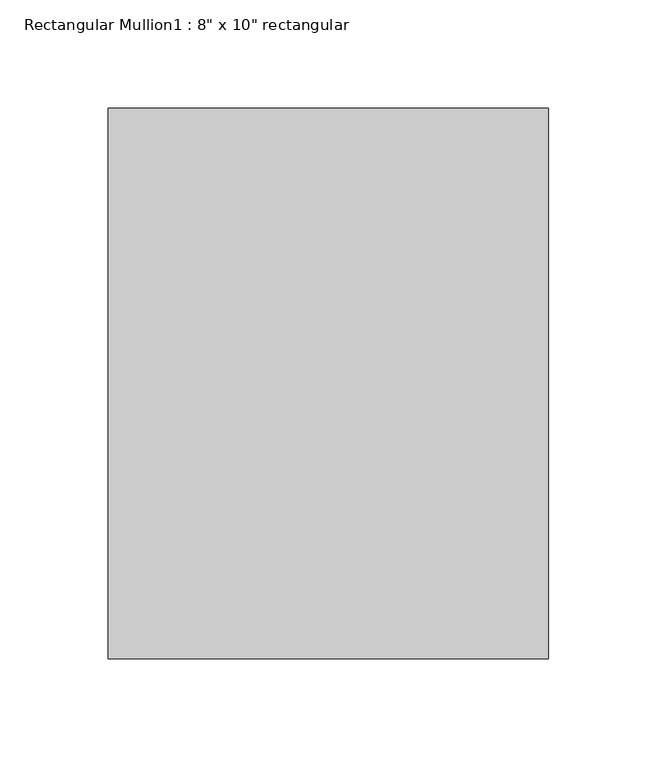
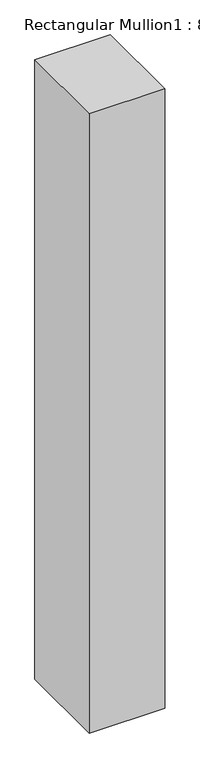
"""IFC4 building model written with IfcOpenShell, lengths in millimetres: member geometry."""

import ifcopenshell
import ifcopenshell.guid

model = None  # the IFC model being written
_history = None  # IfcOwnerHistory: only IFC2X3 demands one
_inside = {}  # id of a spatial element -> (the spatial element, [elements in it])
_under = {}  # id of a project, library or spatial element -> (it, [spatial elements below it])
_declared = {}  # id of a project -> (the project, [libraries it declares])
_typed = {}  # id of a type object -> (the type object, [elements of that type])
_made_of = {}  # id of a material, layer set ... -> (it, [elements and type objects made of it])


def new_model(schema):
    """Start an empty IFC model of exactly this schema.

    Asked for "IFC4X3", IfcOpenShell would pick the latest addendum, in which some entities
    have other attributes; the version numbers below select the first issue.
    IFC2X3 requires an IfcOwnerHistory on every rooted entity: one is made here for all.
    """
    global model, _history
    if schema == "IFC4X3":
        model = ifcopenshell.file(schema_version=(4, 3, 0, 0))
    else:
        model = ifcopenshell.file(schema=schema)
    _inside.clear()
    _under.clear()
    _declared.clear()
    _typed.clear()
    _made_of.clear()
    _history = None
    if model.schema == "IFC2X3":
        org = make("IfcOrganization", Name="unknown")
        user = make(
            "IfcPersonAndOrganization",
            ThePerson=make("IfcPerson", FamilyName="unknown"),
            TheOrganization=org,
        )
        app = make(
            "IfcApplication",
            ApplicationDeveloper=org,
            Version="unknown",
            ApplicationFullName="unknown",
            ApplicationIdentifier="unknown",
        )
        _history = make(
            "IfcOwnerHistory",
            OwningUser=user,
            OwningApplication=app,
            ChangeAction="ADDED",
            CreationDate=0,
        )
    return model


def make(cls, **values):
    """One entity of the class cls with the attributes given. An attribute that is None is left unset."""
    return model.create_entity(
        cls, **{name: value for name, value in values.items() if value is not None}
    )


def rooted(cls, **values):
    """An entity with a GlobalId (a new one), such as an element, a storey or a relation."""
    return make(cls, GlobalId=ifcopenshell.guid.new(), OwnerHistory=_history, **values)


def si_unit(unit_type, name, prefix=None):
    """IfcSIUnit, for example si_unit("LENGTHUNIT", "METRE", prefix="MILLI")."""
    return make("IfcSIUnit", UnitType=unit_type, Prefix=prefix, Name=name)


def assignment(units):
    """IfcUnitAssignment: the units of a project."""
    return None if units is None else make("IfcUnitAssignment", Units=units)


def point(xyz):
    """IfcCartesianPoint."""
    return None if xyz is None else make("IfcCartesianPoint", Coordinates=xyz)


def direction(xyz):
    """IfcDirection."""
    return None if xyz is None else make("IfcDirection", DirectionRatios=xyz)


def frame(location, z_axis=None, x_axis=None):
    """IfcAxis2Placement3D, a coordinate frame: its origin and axes. An axis left out is left unset."""
    return make(
        "IfcAxis2Placement3D",
        Location=point(location),
        Axis=direction(z_axis),
        RefDirection=direction(x_axis),
    )


def origin():
    """The frame at (0, 0, 0) with its axes left unset."""
    return frame((0.0, 0.0, 0.0))


def place(relative_to, where):
    """IfcLocalPlacement: puts the frame where relative to a parent placement (None: the world)."""
    return make(
        "IfcLocalPlacement", PlacementRelTo=relative_to, RelativePlacement=where
    )


def context(
    kind, dimensions, precision=None, world=None, true_north=None, identifier=None
):
    """IfcGeometricRepresentationContext, for example the 3D "Model" context."""
    return make(
        "IfcGeometricRepresentationContext",
        ContextIdentifier=identifier,
        ContextType=kind,
        CoordinateSpaceDimension=dimensions,
        Precision=precision,
        WorldCoordinateSystem=world,
        TrueNorth=true_north,
    )


def project(units=None, contexts=None):
    """IfcProject with its units and contexts."""
    return rooted(
        "IfcProject",
        Name="project",
        RepresentationContexts=contexts,
        UnitsInContext=assignment(units),
    )


def spatial(cls, under=None, at=None, **own):
    """A site, building, storey or space (cls), placed at a placement, below another one or the project."""
    s = rooted(cls, ObjectPlacement=at, **own)
    if under is not None:
        _under.setdefault(under.id(), (under, []))[1].append(s)
    return s


def polyline(points):
    """IfcPolyline through the points."""
    return make("IfcPolyline", Points=[point(p) for p in points])


def outline(outer, holes=None, kind="AREA"):
    """IfcArbitraryClosedProfileDef: a profile drawn as a closed curve; with holes, ...WithVoids."""
    if holes is None:
        return make("IfcArbitraryClosedProfileDef", ProfileType=kind, OuterCurve=outer)
    return make(
        "IfcArbitraryProfileDefWithVoids",
        ProfileType=kind,
        OuterCurve=outer,
        InnerCurves=holes,
    )


def extrude(swept, where, along, depth):
    """IfcExtrudedAreaSolid: the profile swept, set in the frame where, extruded along a direction by depth."""
    return make(
        "IfcExtrudedAreaSolid",
        SweptArea=swept,
        Position=where,
        ExtrudedDirection=direction(along),
        Depth=depth,
    )


def shape(context_of_items, identifier, shape_type, items):
    """IfcShapeRepresentation: the items that make up one representation, for example the "Body"."""
    return make(
        "IfcShapeRepresentation",
        ContextOfItems=context_of_items,
        RepresentationIdentifier=identifier,
        RepresentationType=shape_type,
        Items=items,
    )


def source(mapping_origin, context_of_items, identifier, shape_type, items):
    """IfcRepresentationMap: a shape defined once, which mapped items show again and again."""
    return make(
        "IfcRepresentationMap",
        MappingOrigin=mapping_origin,
        MappedRepresentation=shape(context_of_items, identifier, shape_type, items),
    )


def transform(
    local_origin,
    x_axis=None,
    y_axis=None,
    z_axis=None,
    scale=None,
    scale2=None,
    scale3=None,
    uniform=True,
):
    """IfcCartesianTransformationOperator3D, or its non-uniform kind. x_axis, y_axis, z_axis: its Axis1, 2, 3."""
    if uniform:
        return make(
            "IfcCartesianTransformationOperator3D",
            Axis1=direction(x_axis),
            Axis2=direction(y_axis),
            LocalOrigin=point(local_origin),
            Scale=scale,
            Axis3=direction(z_axis),
        )
    return make(
        "IfcCartesianTransformationOperator3DnonUniform",
        Axis1=direction(x_axis),
        Axis2=direction(y_axis),
        LocalOrigin=point(local_origin),
        Scale=scale,
        Axis3=direction(z_axis),
        Scale2=scale2,
        Scale3=scale3,
    )


def mapped(mapping_source, mapping_target):
    """IfcMappedItem: shows the shape of a source again, moved by a transform."""
    return make(
        "IfcMappedItem", MappingSource=mapping_source, MappingTarget=mapping_target
    )


def made_of(thing, what):
    """Note that an element or type object is made of a material, layer set ...; save() writes the relation."""
    if what is not None:
        _made_of.setdefault(what.id(), (what, []))[1].append(thing)
    return thing


def element(
    cls,
    number,
    at=None,
    inside=None,
    cuts=None,
    type_object=None,
    material=None,
    context=None,
    identifier="Body",
    shape_type=None,
    held_by="IfcProductDefinitionShape",
    body=None,
    shapes=None,
    **own,
):
    """One element of the class cls, such as IfcWall. Its Tag is "e" and its number.

    at: its placement. inside: the storey or other place that contains it. cuts: it is an
    opening in that element (IfcRelVoidsElement). A single representation is given by context,
    identifier, shape_type and body (its items); several are given by shapes. held_by: the class
    of the entity that holds the representations. save() writes the other relations.
    """
    e = rooted(cls, Tag="e%d" % number, ObjectPlacement=at, **own)
    if body is not None:
        shapes = [shape(context, identifier, shape_type, body)]
    if shapes is not None:
        e.Representation = make(held_by, Representations=shapes)
    if inside is not None:
        _inside.setdefault(inside.id(), (inside, []))[1].append(e)
    if cuts is not None:
        rooted(
            "IfcRelVoidsElement", RelatingBuildingElement=cuts, RelatedOpeningElement=e
        )
    if type_object is not None:
        _typed.setdefault(type_object.id(), (type_object, []))[1].append(e)
    return made_of(e, material)


def aggregate(whole, parts):
    """IfcRelAggregates: a whole, such as a stair, and the parts it consists of."""
    return rooted("IfcRelAggregates", RelatingObject=whole, RelatedObjects=parts)


def save(model, path):
    """Write the relations noted so far, then the file.

    IfcRelAggregates (storeys below a building ...), IfcRelContainedInSpatialStructure (elements
    in a storey), IfcRelDefinesByType, IfcRelAssociatesMaterial and IfcRelDeclares: one each for
    every whole, place, type object, material and project.
    """
    for whole, parts in _under.values():
        aggregate(whole, parts)
    for where, things in _inside.values():
        rooted(
            "IfcRelContainedInSpatialStructure",
            RelatedElements=things,
            RelatingStructure=where,
        )
    for kind, things in _typed.values():
        rooted("IfcRelDefinesByType", RelatedObjects=things, RelatingType=kind)
    for what, things in _made_of.values():
        rooted("IfcRelAssociatesMaterial", RelatedObjects=things, RelatingMaterial=what)
    for by, libraries in _declared.values():
        rooted("IfcRelDeclares", RelatingContext=by, RelatedDefinitions=libraries)
    model.write(path)


def member_136c1585(model_context):
    return source(origin(), model_context, "Body", "SweptSolid", [
        extrude(outline(polyline([(0.0, 127.0), (0.0, -127.0), (-203.2, -127.0), (-203.2, 127.0), (0.0, 127.0)])), frame((0.0, 0.0, -1765.3), z_axis=(0.0, 0.0, 1.0), x_axis=(1.0, 0.0, 0.0)), (0.0, 0.0, 1.0), 1765.3),
    ])


if __name__ == "__main__":
    model = new_model("IFC4")
    model_context = context("Model", 3, world=origin())
    ifc_project = project(units=[si_unit("LENGTHUNIT", "METRE", prefix="MILLI")], contexts=[model_context])
    site = spatial("IfcSite", under=ifc_project)
    building = spatial("IfcBuilding", under=site)
    placement = place(None, origin())
    member_shape = member_136c1585(model_context)
    element("IfcMember", 1, ObjectType="Rectangular Mullion1 : 8\" x 10\" rectangular", at=placement, inside=building, context=model_context, shape_type="MappedRepresentation", body=[
        mapped(member_shape, transform((0.0, 0.0, 0.0), x_axis=(1.0, 0.0, 0.0), y_axis=(0.0, 1.0, 0.0), z_axis=(0.0, 0.0, 1.0))),
    ])
    save(model, "model.ifc")

# Revit data of these elements
# Type "Rectangular Mullion1 : 8\" x 10\" rectangular"
#   built-in parameter 1007304 = 0.833333 (stored number, unit not read)
#   built-in parameter 1007301 = 0.333333 (stored number, unit not read)
#   built-in parameter 1007300 = 0.333333 (stored number, unit not read)
# Element 1 (IfcMember, "Rectangular Mullion1 : 8\" x 10\" rectangular")
#   Materials on its faces: "support-frame"
# Materials
#   "support-frame": class "Unassigned", colour RGB 233 233 233, transparency 0, Cost = 0
